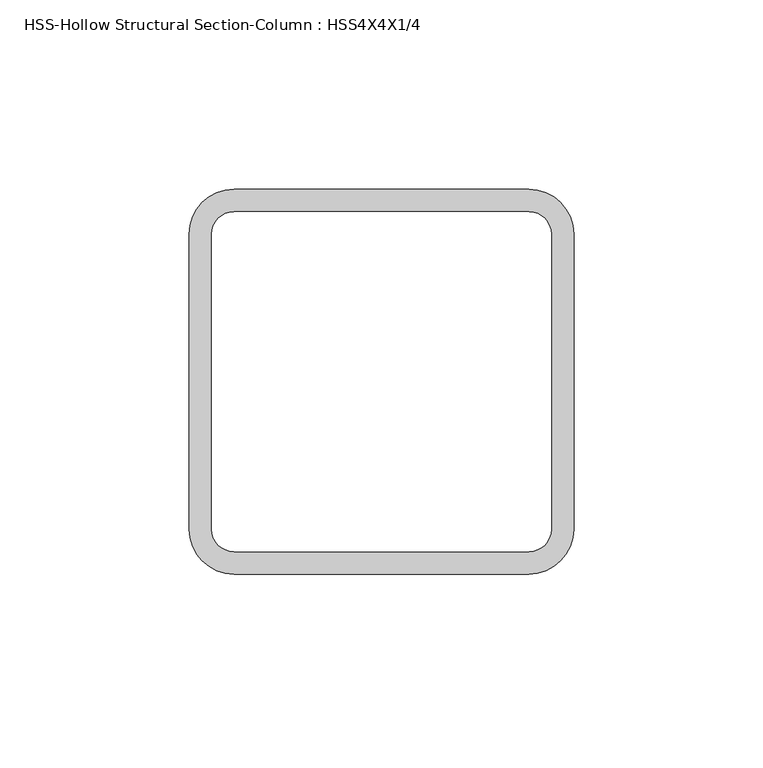
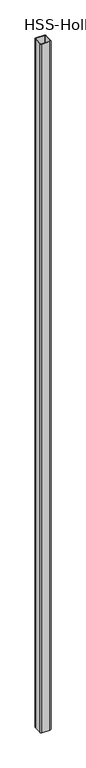
"""IFC4 building model written with IfcOpenShell, lengths in millimetres: column geometry, HSS-Hollow Structural Section-Column : HSS4X4X1/4."""

from ifc_helpers import new_model, si_unit, point, frame_2d, origin, origin_with_axes, place, context, project, spatial, polyline, circle_curve, trimmed, segment, composite_curve, outline, extrude, source, transform, mapped, element, save


def hss_hollow_structural_section_column_hss4x4x1_4_63ca78b6(model_context):
    return source(origin(), model_context, "Body", "SweptSolid", [
        extrude(outline(composite_curve([segment(trimmed(circle_curve(frame_2d((38.9636, 38.9636)), 11.8364), [point((38.9636, 50.8))], [point((50.8, 38.9636))], False, "CARTESIAN"), True, "CONTINUOUS"), segment(polyline([(50.8, 38.9636), (50.8, -38.9636)]), True, "CONTINUOUS"), segment(trimmed(circle_curve(frame_2d((38.9636, -38.9636)), 11.8364), [point((50.8, -38.9636))], [point((38.9636, -50.8))], False, "CARTESIAN"), True, "CONTINUOUS"), segment(polyline([(38.9636, -50.8), (-38.9636, -50.8)]), True, "CONTINUOUS"), segment(trimmed(circle_curve(frame_2d((-38.9636, -38.9636)), 11.8364), [point((-38.9636, -50.8))], [point((-50.8, -38.9636))], False, "CARTESIAN"), True, "CONTINUOUS"), segment(polyline([(-50.8, -38.9636), (-50.8, 38.9636)]), True, "CONTINUOUS"), segment(trimmed(circle_curve(frame_2d((-38.9636, 38.9636)), 11.8364), [point((-50.8, 38.9636))], [point((-38.9636, 50.8))], False, "CARTESIAN"), True, "CONTINUOUS"), segment(polyline([(-38.9636, 50.8), (38.9636, 50.8)]), True, "CONTINUOUS")], self_intersect=False), holes=[composite_curve([segment(polyline([(38.9636, 44.8818), (-38.9636, 44.8818)]), True, "CONTINUOUS"), segment(trimmed(circle_curve(frame_2d((-38.9636, 38.9636)), 5.9182), [point((-38.9636, 44.8818))], [point((-44.8818, 38.9636))], True, "CARTESIAN"), True, "CONTINUOUS"), segment(polyline([(-44.8818, 38.9636), (-44.8818, -38.9636)]), True, "CONTINUOUS"), segment(trimmed(circle_curve(frame_2d((-38.9636, -38.9636)), 5.9182), [point((-44.8818, -38.9636))], [point((-38.9636, -44.8818))], True, "CARTESIAN"), True, "CONTINUOUS"), segment(polyline([(-38.9636, -44.8818), (38.9636, -44.8818)]), True, "CONTINUOUS"), segment(trimmed(circle_curve(frame_2d((38.9636, -38.9636)), 5.9182), [point((38.9636, -44.8818))], [point((44.8818, -38.9636))], True, "CARTESIAN"), True, "CONTINUOUS"), segment(polyline([(44.8818, -38.9636), (44.8818, 38.9636)]), True, "CONTINUOUS"), segment(trimmed(circle_curve(frame_2d((38.9636, 38.9636)), 5.9182), [point((44.8818, 38.9636))], [point((38.9636, 44.8818))], True, "CARTESIAN"), True, "CONTINUOUS")], self_intersect=False)]), origin_with_axes(), (0.0, 0.0, 1.0), 7010.4),
    ])


if __name__ == "__main__":
    model = new_model("IFC4")
    model_context = context("Model", 3, world=origin())
    ifc_project = project(units=[si_unit("LENGTHUNIT", "METRE", prefix="MILLI")], contexts=[model_context])
    site = spatial("IfcSite", under=ifc_project)
    building = spatial("IfcBuilding", under=site)
    placement = place(None, origin())
    hss_hollow_structural_section_column_hss4x4x1_4_shape = hss_hollow_structural_section_column_hss4x4x1_4_63ca78b6(model_context)
    element("IfcColumn", 1, ObjectType="HSS-Hollow Structural Section-Column : HSS4X4X1/4", at=placement, inside=building, context=model_context, shape_type="MappedRepresentation", body=[
        mapped(hss_hollow_structural_section_column_hss4x4x1_4_shape, transform((0.0, 0.0, 0.0), x_axis=(1.0, 0.0, 0.0), y_axis=(0.0, 1.0, 0.0), z_axis=(0.0, 0.0, 1.0))),
    ])
    save(model, "model.ifc")

# Revit data of these elements
# Type "HSS-Hollow Structural Section-Column : HSS4X4X1/4"
#   Assembly Code = "B10"
#   Shape = "Square"
#   W = 12.2
#   Ht = 101.6 mm
#   b = 101.6 mm
#   kr = 11.836 mm
#   t = 5.918 mm
#   A = 0.00217419 m²
#   Structural Material [instance default] = Metal - Steel - ASTM A500 - Grade B - Rectangular and Square
# Element 1 (IfcColumn, "HSS-Hollow Structural Section-Column : HSS4X4X1/4")
#   Materials on its faces: "Metal - Steel - ASTM A500 - Grade B - Rectangular and Square"
# Materials
#   "Metal - Steel - ASTM A500 - Grade B - Rectangular and Square": class "Metal", colour RGB 199 199 199, transparency 0, Cost = 0
